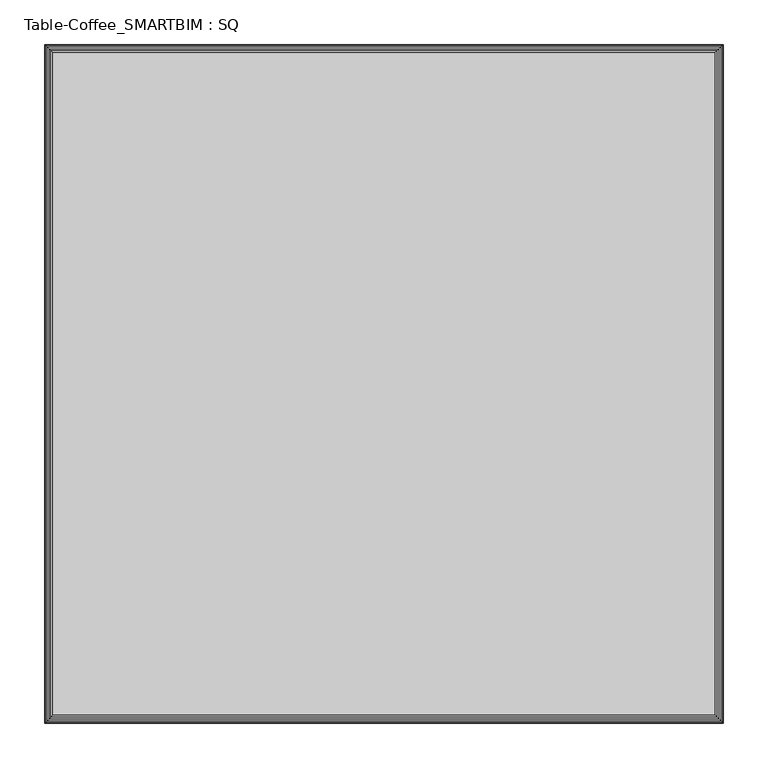
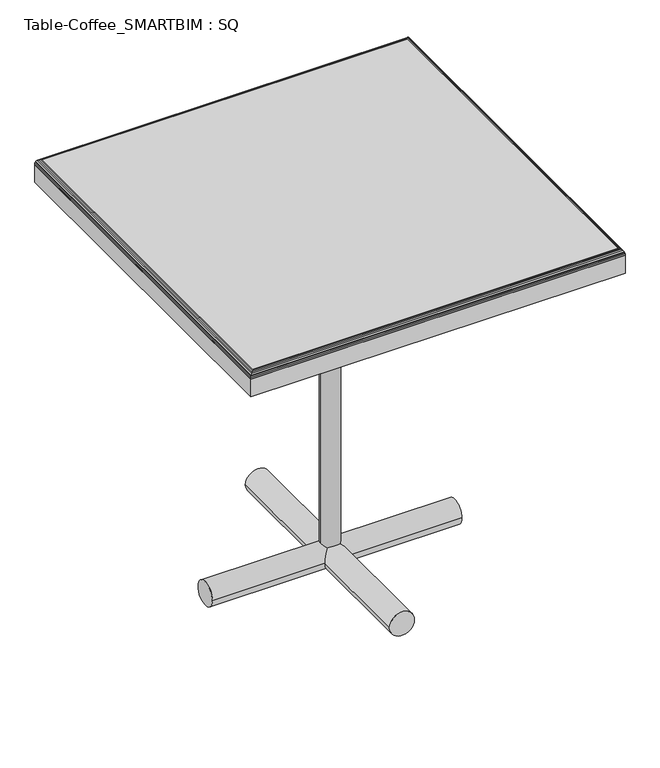
"""IFC4 building model written with IfcOpenShell, lengths in millimetres: furniture geometry, Table-Coffee_SMARTBIM : SQ."""

from ifc_helpers import new_model, si_unit, point, frame, frame_2d, origin, origin_2d, place, context, project, spatial, polyline, circle_curve, ellipse_curve, trimmed, segment, composite_curve, outline, extrude, source, transform, mapped, element, save
from ifc_brep_helpers import plane_surface, cylinder_surface, advanced_brep


def table_coffee_smartbim_sq_4378fec3(model_context):
    return source(origin(), model_context, "Body", "SolidModel", [
        extrude(outline(composite_curve([segment(trimmed(circle_curve(frame_2d((0.0, 25.4)), 25.4), [point((25.4, 25.4))], [point((-25.4, 25.4))], False, "CARTESIAN"), True, "CONTINUOUS"), segment(trimmed(circle_curve(frame_2d((0.0, 25.4)), 25.4), [point((-25.4, 25.4))], [point((25.4, 25.4))], False, "CARTESIAN"), True, "CONTINUOUS")], self_intersect=False)), frame((-254.0, 0.0, 0.0), z_axis=(1.0, 0.0, 0.0), x_axis=(0.0, 1.0, 0.0)), (0.0, 0.0, 1.0), 508.0),
        extrude(outline(composite_curve([segment(trimmed(circle_curve(frame_2d((25.4, 0.0)), 25.4), [point((25.4, -25.4))], [point((25.4, 25.4))], False, "CARTESIAN"), True, "CONTINUOUS"), segment(trimmed(circle_curve(frame_2d((25.4, 0.0)), 25.4), [point((25.4, 25.4))], [point((25.4, -25.4))], False, "CARTESIAN"), True, "CONTINUOUS")], self_intersect=False)), frame((0.0, -254.0, 0.0), z_axis=(0.0, 1.0, 0.0), x_axis=(0.0, 0.0, 1.0)), (0.0, 0.0, 1.0), 508.0),
        extrude(outline(polyline([(381.0, 381.0), (381.0, -381.0), (-381.0, -381.0), (-381.0, 381.0), (381.0, 381.0)])), frame((0.0, 0.0, 723.9), z_axis=(0.0, 0.0, 1.0), x_axis=(1.0, 0.0, 0.0)), (0.0, 0.0, 1.0), 38.1),
        advanced_brep(
        [(-371.5998654, -371.5998654, 774.7), (371.5998654, -371.5998654, 774.7), (371.5998654, 371.5998654, 774.7), (-371.5998654, 371.5998654, 774.7), (381.0, 381.0, 762.0), (381.0, -381.0, 762.0), (-381.0, -381.0, 762.0), (-381.0, 381.0, 762.0), (-381.0, 381.0, 765.2998654), (381.0, 381.0, 765.2998654), (-381.0, -381.0, 765.2998654), (381.0, -381.0, 765.2998654), (-380.6372483, -380.6372483, 767.8860287), (-380.6372483, 380.6372483, 767.8860287), (-373.7616212, 373.7616212, 774.4480533), (-373.7616212, -373.7616212, 774.4480533), (-375.7639185, 375.7639185, 773.7273912), (-375.7639185, -375.7639185, 773.7273912), (-377.8885738, 377.8885738, 772.2866155), (-377.8885738, -377.8885738, 772.2866155), (-379.9102962, 379.9102962, 769.692959), (-379.9102962, -379.9102962, 769.692959), (380.6372483, -380.6372483, 767.8860287), (373.7616212, -373.7616212, 774.4480533), (375.7639185, -375.7639185, 773.7273912), (377.8885738, -377.8885738, 772.2866155), (379.9102962, -379.9102962, 769.692959), (380.6372483, 380.6372483, 767.8860287), (373.7616212, 373.7616212, 774.4480533), (375.7639185, 375.7639185, 773.7273912), (377.8885738, 377.8885738, 772.2866155), (379.9102962, 379.9102962, 769.692959)],
        [
            (0, 1),
            (1, 2),
            (2, 3),
            (3, 0),
            (4, 5),
            (5, 6),
            (6, 7),
            (7, 4),
            (7, 8),
            (8, 9),
            (9, 4),
            (6, 10),
            (10, 8),
            (5, 11),
            (11, 10),
            (9, 11),
            (10, 12, ellipse_curve(frame((-371.5998654, -371.5998654, 765.2998654), z_axis=(-0.7071067811865475, 0.7071067811865475, 0.0), x_axis=(-0.7071067811865474, -0.7071067811865476, 0.0)), 13.2937978, 9.4001346)),
            (12, 13),
            (13, 8, ellipse_curve(frame((-371.5998654, 371.5998654, 765.2998654), z_axis=(-0.7071067811865475, -0.7071067811865475, 0.0), x_axis=(0.7071067811865474, -0.7071067811865476, 0.0)), 13.2937978, 9.4001346)),
            (14, 15),
            (15, 0, ellipse_curve(frame((-371.5998654, -371.5998654, 765.2998654), z_axis=(-0.7071067811865475, 0.7071067811865475, 0.0), x_axis=(-0.7071067811865474, -0.7071067811865476, 0.0)), 13.2937978, 9.4001346)),
            (3, 14, ellipse_curve(frame((-371.5998654, 371.5998654, 765.2998654), z_axis=(-0.7071067811865475, -0.7071067811865475, 0.0), x_axis=(0.7071067811865474, -0.7071067811865476, 0.0)), 13.2937978, 9.4001346)),
            (14, 16, ellipse_curve(frame((-371.5998654, 371.5998654, 765.2998654), z_axis=(-0.7071067811865475, -0.7071067811865475, 0.0), x_axis=(0.7071067811865474, -0.7071067811865476, 0.0)), 13.2937978, 9.4001346)),
            (16, 17),
            (17, 15, ellipse_curve(frame((-371.5998654, -371.5998654, 765.2998654), z_axis=(-0.7071067811865475, 0.7071067811865475, 0.0), x_axis=(-0.7071067811865474, -0.7071067811865476, 0.0)), 13.2937978, 9.4001346)),
            (16, 18, ellipse_curve(frame((-371.5998654, 371.5998654, 765.2998654), z_axis=(-0.7071067811865475, -0.7071067811865475, 0.0), x_axis=(0.7071067811865474, -0.7071067811865476, 0.0)), 13.2937978, 9.4001346)),
            (18, 19),
            (19, 17, ellipse_curve(frame((-371.5998654, -371.5998654, 765.2998654), z_axis=(-0.7071067811865475, 0.7071067811865475, 0.0), x_axis=(-0.7071067811865474, -0.7071067811865476, 0.0)), 13.2937978, 9.4001346)),
            (18, 20, ellipse_curve(frame((-371.5998654, 371.5998654, 765.2998654), z_axis=(-0.7071067811865475, -0.7071067811865475, 0.0), x_axis=(0.7071067811865474, -0.7071067811865476, 0.0)), 13.2937978, 9.4001346)),
            (20, 21),
            (21, 19, ellipse_curve(frame((-371.5998654, -371.5998654, 765.2998654), z_axis=(-0.7071067811865475, 0.7071067811865475, 0.0), x_axis=(-0.7071067811865474, -0.7071067811865476, 0.0)), 13.2937978, 9.4001346)),
            (12, 21, ellipse_curve(frame((-371.5998654, -371.5998654, 765.2998654), z_axis=(-0.7071067811865475, 0.7071067811865475, 0.0), x_axis=(-0.7071067811865474, -0.7071067811865476, 0.0)), 13.2937978, 9.4001346)),
            (20, 13, ellipse_curve(frame((-371.5998654, 371.5998654, 765.2998654), z_axis=(-0.7071067811865475, -0.7071067811865475, 0.0), x_axis=(0.7071067811865474, -0.7071067811865476, 0.0)), 13.2937978, 9.4001346)),
            (11, 22, ellipse_curve(frame((371.5998654, -371.5998654, 765.2998654), z_axis=(-0.7071067811865475, -0.7071067811865475, 0.0), x_axis=(0.7071067811865476, -0.7071067811865474, 0.0)), 13.2937978, 9.4001346)),
            (22, 12),
            (15, 23),
            (23, 1, ellipse_curve(frame((371.5998654, -371.5998654, 765.2998654), z_axis=(-0.7071067811865475, -0.7071067811865475, 0.0), x_axis=(0.7071067811865476, -0.7071067811865474, 0.0)), 13.2937978, 9.4001346)),
            (17, 24),
            (24, 23, ellipse_curve(frame((371.5998654, -371.5998654, 765.2998654), z_axis=(-0.7071067811865475, -0.7071067811865475, 0.0), x_axis=(0.7071067811865476, -0.7071067811865474, 0.0)), 13.2937978, 9.4001346)),
            (19, 25),
            (25, 24, ellipse_curve(frame((371.5998654, -371.5998654, 765.2998654), z_axis=(-0.7071067811865475, -0.7071067811865475, 0.0), x_axis=(0.7071067811865476, -0.7071067811865474, 0.0)), 13.2937978, 9.4001346)),
            (21, 26),
            (26, 25, ellipse_curve(frame((371.5998654, -371.5998654, 765.2998654), z_axis=(-0.7071067811865475, -0.7071067811865475, 0.0), x_axis=(0.7071067811865476, -0.7071067811865474, 0.0)), 13.2937978, 9.4001346)),
            (22, 26, ellipse_curve(frame((371.5998654, -371.5998654, 765.2998654), z_axis=(-0.7071067811865475, -0.7071067811865475, 0.0), x_axis=(0.7071067811865476, -0.7071067811865474, 0.0)), 13.2937978, 9.4001346)),
            (9, 27, ellipse_curve(frame((371.5998654, 371.5998654, 765.2998654), z_axis=(0.7071067811865475, -0.7071067811865475, 0.0), x_axis=(0.7071067811865474, 0.7071067811865476, 0.0)), 13.2937978, 9.4001346)),
            (27, 22),
            (23, 28),
            (28, 2, ellipse_curve(frame((371.5998654, 371.5998654, 765.2998654), z_axis=(0.7071067811865475, -0.7071067811865475, 0.0), x_axis=(0.7071067811865474, 0.7071067811865476, 0.0)), 13.2937978, 9.4001346)),
            (24, 29),
            (29, 28, ellipse_curve(frame((371.5998654, 371.5998654, 765.2998654), z_axis=(0.7071067811865475, -0.7071067811865475, 0.0), x_axis=(0.7071067811865474, 0.7071067811865476, 0.0)), 13.2937978, 9.4001346)),
            (25, 30),
            (30, 29, ellipse_curve(frame((371.5998654, 371.5998654, 765.2998654), z_axis=(0.7071067811865475, -0.7071067811865475, 0.0), x_axis=(0.7071067811865474, 0.7071067811865476, 0.0)), 13.2937978, 9.4001346)),
            (26, 31),
            (31, 30, ellipse_curve(frame((371.5998654, 371.5998654, 765.2998654), z_axis=(0.7071067811865475, -0.7071067811865475, 0.0), x_axis=(0.7071067811865474, 0.7071067811865476, 0.0)), 13.2937978, 9.4001346)),
            (27, 31, ellipse_curve(frame((371.5998654, 371.5998654, 765.2998654), z_axis=(0.7071067811865475, -0.7071067811865475, 0.0), x_axis=(0.7071067811865474, 0.7071067811865476, 0.0)), 13.2937978, 9.4001346)),
            (13, 27),
            (28, 14),
            (29, 16),
            (30, 18),
            (31, 20),
        ],
        [
            plane_surface(frame((-381.0, 381.0, 774.7), z_axis=(0.0, 0.0, 1.0), x_axis=(-1.0, 0.0, 0.0))),
            plane_surface(frame((-381.0, 381.0, 762.0), z_axis=(0.0, 0.0, -1.0), x_axis=(1.0, 0.0, 0.0))),
            plane_surface(frame((381.0, 381.0, 774.7), z_axis=(0.0, 1.0, 0.0), x_axis=(0.0, 0.0, -1.0))),
            plane_surface(frame((-381.0, 381.0, 774.7), z_axis=(-1.0, 0.0, 0.0), x_axis=(0.0, 0.0, -1.0))),
            plane_surface(frame((-381.0, -381.0, 774.7), z_axis=(0.0, -1.0, 0.0), x_axis=(0.0, 0.0, -1.0))),
            plane_surface(frame((381.0, -381.0, 774.7), z_axis=(1.0, 0.0, 0.0), x_axis=(0.0, 0.0, -1.0))),
            cylinder_surface(frame((-371.5998654, 381.0, 765.2998654), z_axis=(0.0, -1.0, 0.0), x_axis=(1.0, 0.0, 0.0)), 9.4001346),
            cylinder_surface(frame((-381.0, -371.5998654, 765.2998654), z_axis=(1.0, 0.0, 0.0), x_axis=(0.0, 1.0, 0.0)), 9.4001346),
            cylinder_surface(frame((371.5998654, -381.0, 765.2998654), z_axis=(0.0, 1.0, 0.0), x_axis=(-1.0, 0.0, 0.0)), 9.4001346),
            cylinder_surface(frame((381.0, 371.5998654, 765.2998654), z_axis=(-1.0, 0.0, 0.0), x_axis=(0.0, -1.0, 0.0)), 9.4001346),
        ],
        [
            (0, [[1, 2, 3, 4]]),
            (1, [[5, 6, 7, 8]]),
            (2, [[-8, 9, 10, 11]]),
            (3, [[-7, 12, 13, -9]]),
            (4, [[-6, 14, 15, -12]]),
            (5, [[-5, -11, 16, -14]]),
            (6, [[17, 18, 19, -13]]),
            (6, [[20, 21, -4, 22]]),
            (6, [[-20, 23, 24, 25]]),
            (6, [[-24, 26, 27, 28]]),
            (6, [[-27, 29, 30, 31]]),
            (6, [[-18, 32, -30, 33]]),
            (7, [[-17, -15, 34, 35]]),
            (7, [[-21, 36, 37, -1]]),
            (7, [[-25, 38, 39, -36]]),
            (7, [[-28, 40, 41, -38]]),
            (7, [[-31, 42, 43, -40]]),
            (7, [[-32, -35, 44, -42]]),
            (8, [[-34, -16, 45, 46]]),
            (8, [[-37, 47, 48, -2]]),
            (8, [[-39, 49, 50, -47]]),
            (8, [[-41, 51, 52, -49]]),
            (8, [[-43, 53, 54, -51]]),
            (8, [[-44, -46, 55, -53]]),
            (9, [[-19, 56, -45, -10]]),
            (9, [[-22, -3, -48, 57]]),
            (9, [[-23, -57, -50, 58]]),
            (9, [[-26, -58, -52, 59]]),
            (9, [[-29, -59, -54, 60]]),
            (9, [[-33, -60, -55, -56]]),
        ],
    ),
        extrude(outline(polyline([(76.2, 76.2), (76.2, -76.2), (-76.2, -76.2), (-76.2, 76.2), (76.2, 76.2)])), frame((0.0, 0.0, 755.65), z_axis=(0.0, 0.0, 1.0), x_axis=(1.0, 0.0, 0.0)), (0.0, 0.0, 1.0), 6.35),
        extrude(outline(composite_curve([segment(trimmed(circle_curve(origin_2d(), 19.05), [point((-19.05, 0.0))], [point((19.05, 0.0))], False, "CARTESIAN"), True, "CONTINUOUS"), segment(trimmed(circle_curve(origin_2d(), 19.05), [point((19.05, 0.0))], [point((-19.05, 0.0))], False, "CARTESIAN"), True, "CONTINUOUS")], self_intersect=False)), frame((0.0, 0.0, 24.2070278), z_axis=(0.0, 0.0, 1.0), x_axis=(1.0, 0.0, 0.0)), (0.0, 0.0, 1.0), 731.4429722),
    ])


if __name__ == "__main__":
    model = new_model("IFC4")
    model_context = context("Model", 3, world=origin())
    ifc_project = project(units=[si_unit("LENGTHUNIT", "METRE", prefix="MILLI")], contexts=[model_context])
    site = spatial("IfcSite", under=ifc_project)
    building = spatial("IfcBuilding", under=site)
    placement = place(None, origin())
    table_coffee_smartbim_sq_shape = table_coffee_smartbim_sq_4378fec3(model_context)
    element("IfcFurniture", 1, ObjectType="Table-Coffee_SMARTBIM : SQ", at=placement, inside=building, context=model_context, shape_type="MappedRepresentation", body=[
        mapped(table_coffee_smartbim_sq_shape, transform((0.0, 0.0, 0.0), x_axis=(1.0, 0.0, 0.0), y_axis=(0.0, 1.0, 0.0), z_axis=(0.0, 0.0, 1.0))),
    ])
    save(model, "model.ifc")

# Revit data of these elements
# Type "Table-Coffee_SMARTBIM : SQ"
#   Subcategory = "Table\r\n"
#   SmartBIM Object Created By = "SMARTBIM, LLC"
#   Manufacturer = "SMARTBIM"
#   Assembly Code = "E2020200"
#   95 CSI = "12500"
#   04 CSI = "12 50 00"
#   table cloth = 0' - 1 1/2"
#   Width = 2' - 6"
#   SmartBIM Object Version = 3
#   Height = 2' - 6"
#   Depth = 2' - 6"
#   Default Elevation = 4' - 0"
#   white cloth_parameter = WOOD-OAKFIRE
#   Table Unit = MET
#   Glide = none
#   Glass = none
# Element 1 (IfcFurniture, "Table-Coffee_SMARTBIM : SQ")
#   Materials on its faces: "WOOD-OAKFIRE", "MET"
# Materials
#   "WOOD-OAKFIRE": class "Wood", colour RGB 198 202 183, transparency 0, Description = "Generic wood", Cost = 0
#   "MET": class "Metal", colour RGB 189 187 185, transparency 0
